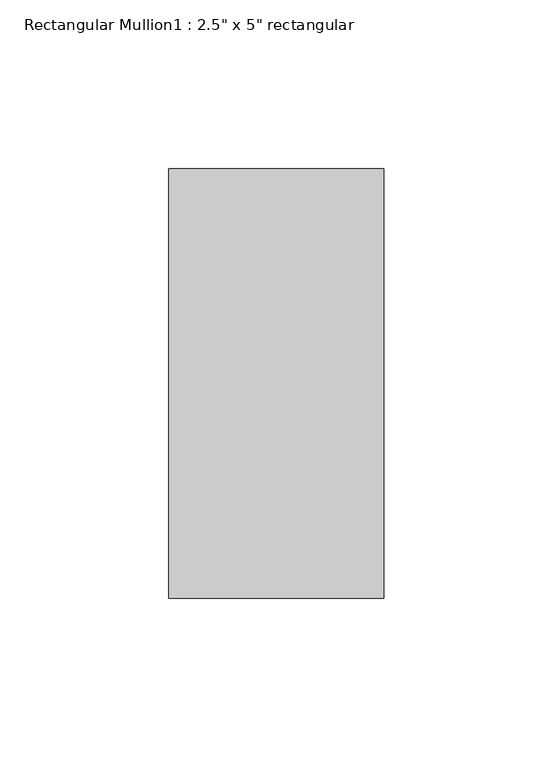
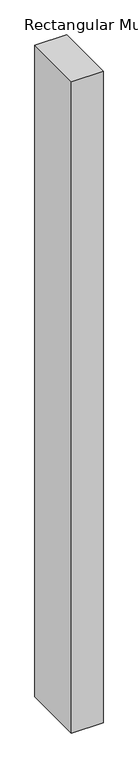
"""IFC4 building model written with IfcOpenShell, lengths in millimetres: member geometry."""

from ifc_helpers import new_model, si_unit, frame, origin, place, context, project, spatial, polyline, outline, extrude, source, transform, mapped, element, save


def member_5e02c13a(model_context):
    return source(origin(), model_context, "Body", "SweptSolid", [
        extrude(outline(polyline([(0.0, 63.5), (0.0, -63.5), (-63.5, -63.5), (-63.5, 63.5), (0.0, 63.5)])), frame((0.0, 0.0, -1383.5673076), z_axis=(0.0, 0.0, 1.0), x_axis=(1.0, 0.0, 0.0)), (0.0, 0.0, 1.0), 1383.5673076),
    ])


if __name__ == "__main__":
    model = new_model("IFC4")
    model_context = context("Model", 3, world=origin())
    ifc_project = project(units=[si_unit("LENGTHUNIT", "METRE", prefix="MILLI")], contexts=[model_context])
    site = spatial("IfcSite", under=ifc_project)
    building = spatial("IfcBuilding", under=site)
    placement = place(None, origin())
    member_shape = member_5e02c13a(model_context)
    element("IfcMember", 1, ObjectType="Rectangular Mullion1 : 2.5\" x 5\" rectangular", at=placement, inside=building, context=model_context, shape_type="MappedRepresentation", body=[
        mapped(member_shape, transform((0.0, 0.0, 0.0), x_axis=(1.0, 0.0, 0.0), y_axis=(0.0, 1.0, 0.0), z_axis=(0.0, 0.0, 1.0))),
    ])
    save(model, "model.ifc")

# Revit data of these elements
# Type "Rectangular Mullion1 : 2.5\" x 5\" rectangular"
#   built-in parameter 1007304 = 0.416667 (stored number, unit not read)
#   built-in parameter 1007301 = 0.104167 (stored number, unit not read)
#   built-in parameter 1007300 = 0.104167 (stored number, unit not read)
# Element 1 (IfcMember, "Rectangular Mullion1 : 2.5\" x 5\" rectangular")
#   Materials on its faces: "support-frame"
# Materials
#   "support-frame": class "Unassigned", colour RGB 233 233 233, transparency 0, Cost = 0
